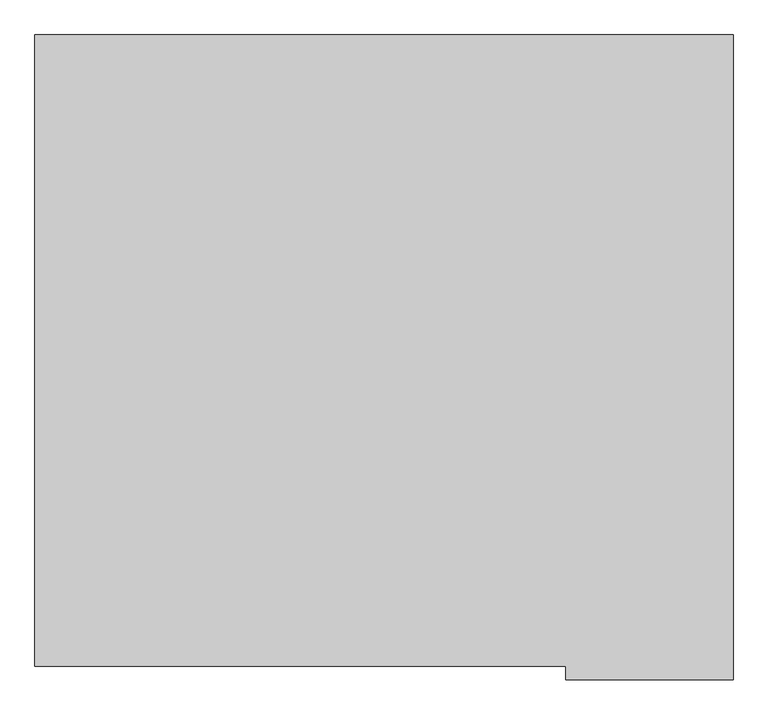
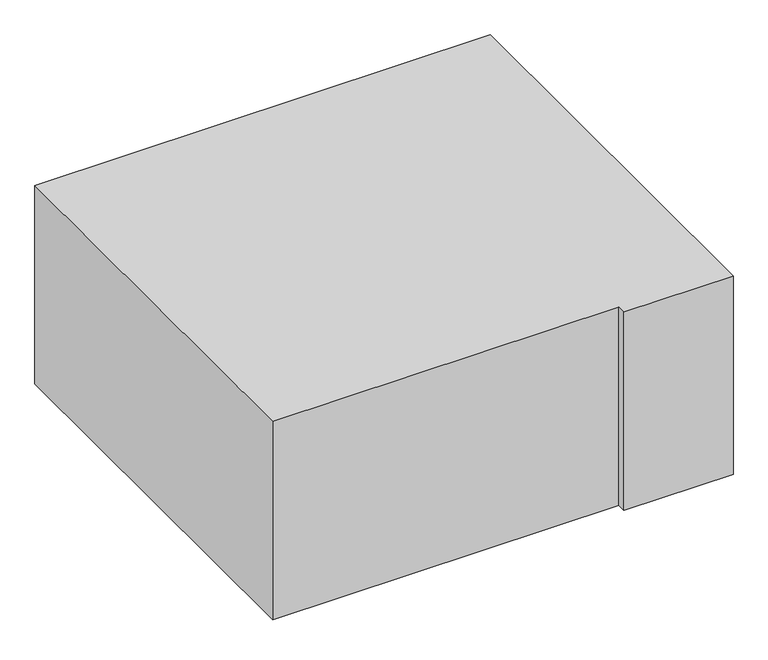
"""IFC4 building model written with IfcOpenShell, lengths in millimetres: proxy geometry, 0_3d_modell."""

from ifc_helpers import new_model, si_unit, origin, origin_with_axes, place, context, project, spatial, polyline, outline, extrude, source, transform, mapped, element, save


def generic_models_fe85dac7(model_context):
    return source(origin(), model_context, "Body", "SweptSolid", [
        extrude(outline(polyline([(6250.0, 5772.0), (6250.0, 0.0), (4750.0, 0.0), (4750.0, 122.0), (0.0, 122.0), (0.0, 5772.0), (6250.0, 5772.0)])), origin_with_axes(), (0.0, 0.0, 1.0), 2880.0),
    ])


if __name__ == "__main__":
    model = new_model("IFC4")
    model_context = context("Model", 3, world=origin())
    ifc_project = project(units=[si_unit("LENGTHUNIT", "METRE", prefix="MILLI")], contexts=[model_context])
    site = spatial("IfcSite", under=ifc_project)
    building = spatial("IfcBuilding", under=site)
    placement = place(None, origin())
    generic_models_shape = generic_models_fe85dac7(model_context)
    element("IfcBuildingElementProxy", 1, Name="0_3d_modell", ObjectType="0_3d_modell", at=placement, inside=building, context=model_context, shape_type="MappedRepresentation", body=[
        mapped(generic_models_shape, transform((0.0, 0.0, 0.0), x_axis=(1.0, 0.0, 0.0), y_axis=(0.0, 1.0, 0.0), z_axis=(0.0, 0.0, 1.0))),
    ])
    save(model, "model.ifc")

# Revit data of these elements
# Element 1 (IfcBuildingElementProxy, "0_3d_modell")
#   Materials on its faces: "*1"
# Materials
#   "*1": class "Unassigned", colour RGB 175 175 175, transparency 0
